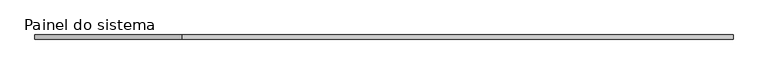
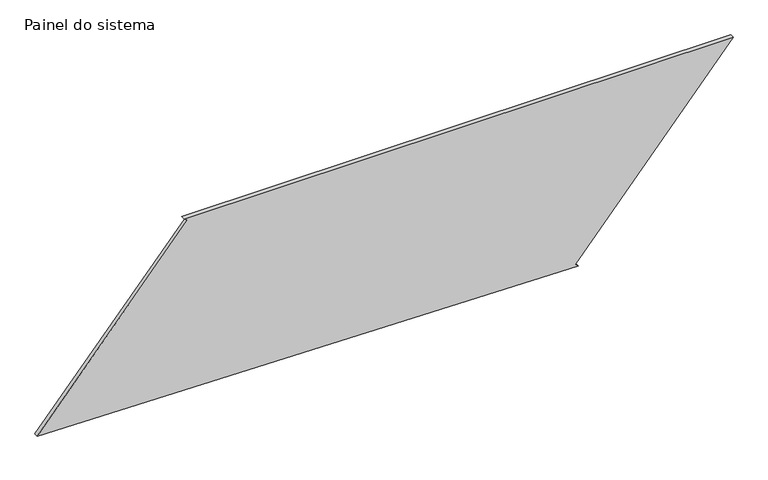
"""IFC4 building model written with IfcOpenShell, lengths in millimetres: plate geometry, Painel do sistema : Envidraçado."""

from ifc_helpers import new_model, si_unit, frame, origin, place, context, project, spatial, polyline, outline, extrude, source, transform, mapped, element, save


def painel_do_sistema_4dea8d27(model_context):
    return source(origin(), model_context, "Body", "SweptSolid", [
        extrude(outline(polyline([(0.0, 1178.0517638), (16.2242617, 1159.0314239), (1146.0103574, 2122.7337216), (1146.0103574, -1225.8249079), (1129.7860957, -1206.8045679), (56.0063352, -2122.7337216), (0.0, 1178.0517638)])), frame((0.0, 24.5, 0.0), z_axis=(0.0, 1.0, 0.0), x_axis=(0.0, 0.0, 1.0)), (0.0, 0.0, 1.0), 25.0),
    ])


if __name__ == "__main__":
    model = new_model("IFC4")
    model_context = context("Model", 3, world=origin())
    ifc_project = project(units=[si_unit("LENGTHUNIT", "METRE", prefix="MILLI")], contexts=[model_context])
    site = spatial("IfcSite", under=ifc_project)
    building = spatial("IfcBuilding", under=site)
    placement = place(None, origin())
    painel_do_sistema_shape = painel_do_sistema_4dea8d27(model_context)
    element("IfcPlate", 1, ObjectType="Painel do sistema : Envidraçado", at=placement, inside=building, context=model_context, shape_type="MappedRepresentation", body=[
        mapped(painel_do_sistema_shape, transform((0.0, 0.0, 0.0), x_axis=(1.0, 0.0, 0.0), y_axis=(0.0, 1.0, 0.0), z_axis=(0.0, 0.0, 1.0))),
    ])
    save(model, "model.ifc")

# Revit data of these elements
# Type "Painel do sistema : Envidraçado"
#   Construction Type Id = "GSP4R"
#   Analytic Construction = "Vidraça única Pilkington 1/8 pol"
#   Visual Light Transmittance = 0.9
#   Solar Heat Gain Coefficient = 0.86
#   Heat Transfer Coefficient (U) = 6.7069 W/(m²·K)
# Element 1 (IfcPlate, "Painel do sistema : Envidraçado")
#   Materials on its faces: "Vidro"
# Materials
#   "Vidro": class "Vidro", colour RGB 0 128 192, transparency 0.9, Description = "Vidro de sílica", Cost = 0
